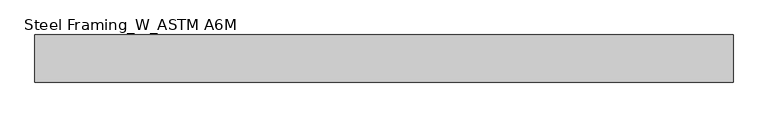
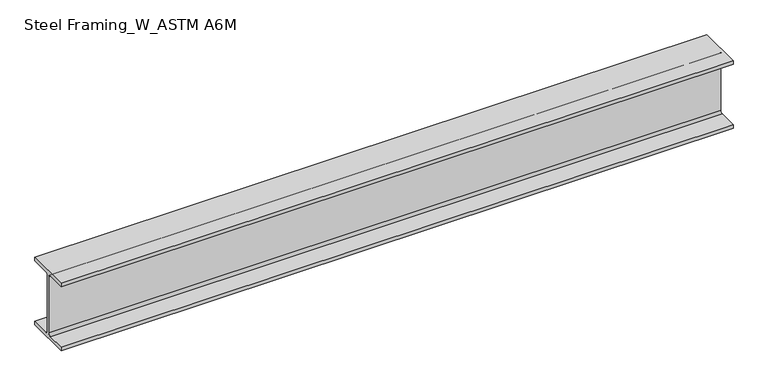
"""IFC4 building model written with IfcOpenShell, lengths in millimetres: beam geometry, Steel Framing_W_ASTM A6M : H_SB_AR_S02_W200x31.3_B6."""

from ifc_helpers import new_model, si_unit, point, frame, frame_2d, origin, place, context, project, spatial, polyline, circle_curve, trimmed, segment, composite_curve, outline, extrude, source, transform, mapped, element, save


def steel_framing_w_astm_a6m_2a4520e6(model_context):
    return source(origin(), model_context, "Body", "SweptSolid", [
        extrude(outline(composite_curve([segment(polyline([(67.0, -94.8), (67.0, -105.0), (-67.0, -105.0), (-67.0, -94.8), (-10.775, -94.8)]), True, "CONTINUOUS"), segment(trimmed(circle_curve(frame_2d((-10.775, -87.2)), 7.6), [point((-10.775, -94.8))], [point((-3.175, -87.2))], True, "CARTESIAN"), True, "CONTINUOUS"), segment(polyline([(-3.175, -87.2), (-3.175, 87.2)]), True, "CONTINUOUS"), segment(trimmed(circle_curve(frame_2d((-10.775, 87.2)), 7.6), [point((-3.175, 87.2))], [point((-10.775, 94.8))], True, "CARTESIAN"), True, "CONTINUOUS"), segment(polyline([(-10.775, 94.8), (-67.0, 94.8), (-67.0, 105.0), (67.0, 105.0), (67.0, 94.8), (10.775, 94.8)]), True, "CONTINUOUS"), segment(trimmed(circle_curve(frame_2d((10.775, 87.2)), 7.6), [point((10.775, 94.8))], [point((3.175, 87.2))], True, "CARTESIAN"), True, "CONTINUOUS"), segment(polyline([(3.175, 87.2), (3.175, -87.2)]), True, "CONTINUOUS"), segment(trimmed(circle_curve(frame_2d((10.775, -87.2)), 7.6), [point((3.175, -87.2))], [point((10.775, -94.8))], True, "CARTESIAN"), True, "CONTINUOUS"), segment(polyline([(10.775, -94.8), (67.0, -94.8)]), True, "CONTINUOUS")], self_intersect=False)), frame((-992.5, 0.0, 0.0), z_axis=(1.0, 0.0, 0.0), x_axis=(0.0, 1.0, 0.0)), (0.0, 0.0, 1.0), 1985.0),
    ])


if __name__ == "__main__":
    model = new_model("IFC4")
    model_context = context("Model", 3, world=origin())
    ifc_project = project(units=[si_unit("LENGTHUNIT", "METRE", prefix="MILLI")], contexts=[model_context])
    site = spatial("IfcSite", under=ifc_project)
    building = spatial("IfcBuilding", under=site)
    placement = place(None, origin())
    steel_framing_w_astm_a6m_shape = steel_framing_w_astm_a6m_2a4520e6(model_context)
    element("IfcBeam", 1, ObjectType="Steel Framing_W_ASTM A6M : H_SB_AR_S02_W200x31.3_B6", at=placement, inside=building, context=model_context, shape_type="MappedRepresentation", body=[
        mapped(steel_framing_w_astm_a6m_shape, transform((0.0, 0.0, 0.0), x_axis=(1.0, 0.0, 0.0), y_axis=(0.0, 1.0, 0.0), z_axis=(0.0, 0.0, 1.0))),
    ])
    save(model, "model.ifc")

# Revit data of these elements
# Type "Steel Framing_W_ASTM A6M : H_SB_AR_S02_W200x31.3_B6"
#   Type Mark = "B6"
#   Section Name Key = "W8x21"
#   Width = 13.4 cm
#   Web Thickness = 0.635 cm
#   Web Fillet = 0.76 cm
#   Warping Constant = 40800.0 cm⁶
#   Torsional Moment of Inertia = 11.70 cm⁴
#   Section Area = 39.7 cm²
#   Plastic Modulus weak axis = 93.2 cm³
#   Plastic Modulus strong axis = 334.0 cm³
#   Perimeter = 0.93 m²/m
#   Nominal Weight = 31.30 kgf/m
#   Moment of Inertia weak axis = 407.00 cm⁴
#   Moment of Inertia strong axis = 3130.00 cm⁴
#   Height = 21.0 cm
#   Flange Thickness = 1.02 cm
#   Elastic Modulus weak axis = 60.8 cm³
#   Elastic Modulus strong axis = 298.0 cm³
#   Centroid Vertical = 10.5 cm
#   Centroid Horizontal = 6.7 cm
#   Length [instance default] = 1500 mm
#   Structural Material [instance default] = Steel, 45-345
#   Bolt Spacing = 0
#   Assembly Code = ""
# Element 1 (IfcBeam, "Steel Framing_W_ASTM A6M : H_SB_AR_S02_W200x31.3_B6")
#   Materials on its faces: "Steel, 45-345"
# Materials
#   "Steel, 45-345": class "Metal", colour RGB 189 187 185, transparency 0, Description = "Steel 345 MPa", Cost = 0
